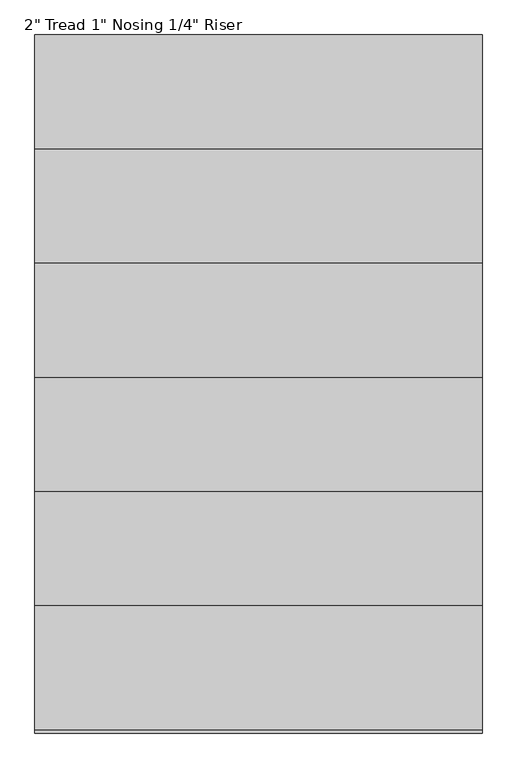
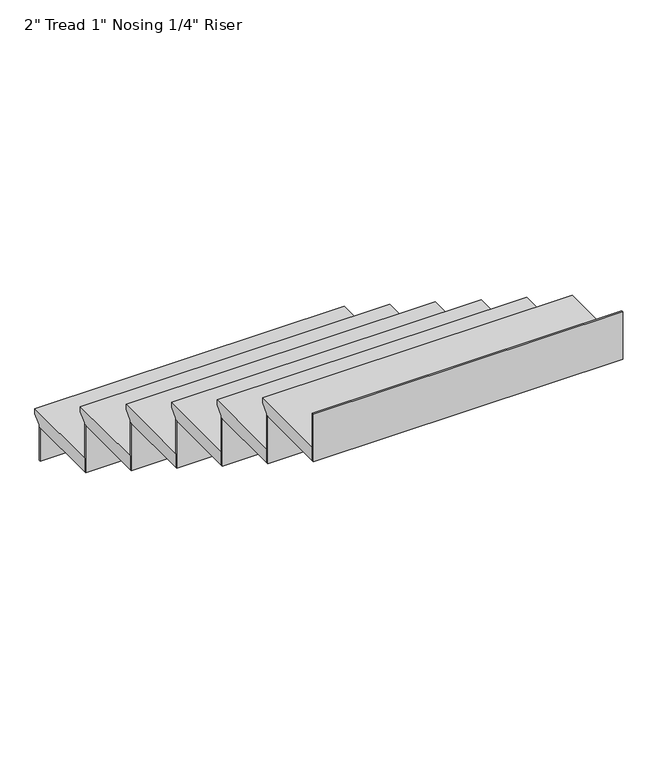
"""IFC4 building model written with IfcOpenShell, lengths in millimetres: stair flight geometry."""

from ifc_helpers import new_model, si_unit, frame, origin, place, context, project, spatial, polyline, outline, extrude, source, transform, mapped, element, save


def stair_flight_3c370561(model_context):
    return source(origin(), model_context, "Body", "SweptSolid", [
        extrude(outline(polyline([(16835.0111033, 2000.25), (17139.8111033, 2000.25), (17139.8111033, 1981.2), (17114.4111033, 1955.8), (17114.4111033, 1949.45), (16835.0111033, 1949.45), (16835.0111033, 2000.25)])), frame((-1579.5625, 0.0, 0.0), z_axis=(1.0, 0.0, 0.0), x_axis=(0.0, 1.0, 0.0)), (0.0, 0.0, 1.0), 1095.3438024),
        extrude(outline(polyline([(-1579.5625, 17108.0611033), (-1579.5625, 17114.4111033), (-484.2186975, 17114.4111033), (-484.2186975, 17108.0611033), (-1579.5625, 17108.0611033)])), frame((0.0, 0.0, 1822.45), z_axis=(0.0, 0.0, 1.0), x_axis=(1.0, 0.0, 0.0)), (0.0, 0.0, 1.0), 127.0),
        extrude(outline(polyline([(-1579.5625, 16828.6611033), (-1579.5625, 16835.0111033), (-484.2186975, 16835.0111033), (-484.2186975, 16828.6611033), (-1579.5625, 16828.6611033)])), frame((0.0, 0.0, 1949.45), z_axis=(0.0, 0.0, 1.0), x_axis=(1.0, 0.0, 0.0)), (0.0, 0.0, 1.0), 177.8),
        extrude(outline(polyline([(16555.6111033, 2178.05), (16860.4111033, 2178.05), (16860.4111033, 2159.0), (16835.0111033, 2133.6), (16835.0111033, 2127.25), (16555.6111033, 2127.25), (16555.6111033, 2178.05)])), frame((-1579.5625, 0.0, 0.0), z_axis=(1.0, 0.0, 0.0), x_axis=(0.0, 1.0, 0.0)), (0.0, 0.0, 1.0), 1095.3438024),
        extrude(outline(polyline([(-1579.5625, 16549.2611033), (-1579.5625, 16555.6111033), (-484.2186975, 16555.6111033), (-484.2186975, 16549.2611033), (-1579.5625, 16549.2611033)])), frame((0.0, 0.0, 2127.25), z_axis=(0.0, 0.0, 1.0), x_axis=(1.0, 0.0, 0.0)), (0.0, 0.0, 1.0), 177.8),
        extrude(outline(polyline([(16276.2111033, 2355.85), (16581.0111033, 2355.85), (16581.0111033, 2336.8), (16555.6111033, 2311.4), (16555.6111033, 2305.05), (16276.2111033, 2305.05), (16276.2111033, 2355.85)])), frame((-1579.5625, 0.0, 0.0), z_axis=(1.0, 0.0, 0.0), x_axis=(0.0, 1.0, 0.0)), (0.0, 0.0, 1.0), 1095.3438024),
        extrude(outline(polyline([(-1579.5625, 16269.8611033), (-1579.5625, 16276.2111033), (-484.2186975, 16276.2111033), (-484.2186975, 16269.8611033), (-1579.5625, 16269.8611033)])), frame((0.0, 0.0, 2305.05), z_axis=(0.0, 0.0, 1.0), x_axis=(1.0, 0.0, 0.0)), (0.0, 0.0, 1.0), 177.8),
        extrude(outline(polyline([(15996.8111033, 2533.65), (16301.6111033, 2533.65), (16301.6111033, 2514.6), (16276.2111033, 2489.2), (16276.2111033, 2482.85), (15996.8111033, 2482.85), (15996.8111033, 2533.65)])), frame((-1579.5625, 0.0, 0.0), z_axis=(1.0, 0.0, 0.0), x_axis=(0.0, 1.0, 0.0)), (0.0, 0.0, 1.0), 1095.3438024),
        extrude(outline(polyline([(-1579.5625, 15990.4611033), (-1579.5625, 15996.8111033), (-484.2186975, 15996.8111033), (-484.2186975, 15990.4611033), (-1579.5625, 15990.4611033)])), frame((0.0, 0.0, 2482.85), z_axis=(0.0, 0.0, 1.0), x_axis=(1.0, 0.0, 0.0)), (0.0, 0.0, 1.0), 177.8),
        extrude(outline(polyline([(15717.4111033, 2711.45), (16022.2111033, 2711.45), (16022.2111033, 2692.4), (15996.8111033, 2667.0), (15996.8111033, 2660.65), (15717.4111033, 2660.65), (15717.4111033, 2711.45)])), frame((-1579.5625, 0.0, 0.0), z_axis=(1.0, 0.0, 0.0), x_axis=(0.0, 1.0, 0.0)), (0.0, 0.0, 1.0), 1095.3438024),
        extrude(outline(polyline([(-1579.5625, 15711.0611033), (-1579.5625, 15717.4111033), (-484.2186975, 15717.4111033), (-484.2186975, 15711.0611033), (-1579.5625, 15711.0611033)])), frame((0.0, 0.0, 2660.65), z_axis=(0.0, 0.0, 1.0), x_axis=(1.0, 0.0, 0.0)), (0.0, 0.0, 1.0), 177.8),
        extrude(outline(polyline([(-1579.5625, 15431.6611033), (-1579.5625, 15438.0111033), (-484.2186975, 15438.0111033), (-484.2186975, 15431.6611033), (-1579.5625, 15431.6611033)])), frame((0.0, 0.0, 2838.45), z_axis=(0.0, 0.0, 1.0), x_axis=(1.0, 0.0, 0.0)), (0.0, 0.0, 1.0), 177.8),
        extrude(outline(polyline([(15438.0111033, 2889.25), (15742.8111033, 2889.25), (15742.8111033, 2870.2), (15717.4111033, 2844.8), (15717.4111033, 2838.45), (15438.0111033, 2838.45), (15438.0111033, 2889.25)])), frame((-1579.5625, 0.0, 0.0), z_axis=(1.0, 0.0, 0.0), x_axis=(0.0, 1.0, 0.0)), (0.0, 0.0, 1.0), 1095.3438024),
    ])


if __name__ == "__main__":
    model = new_model("IFC4")
    model_context = context("Model", 3, world=origin())
    ifc_project = project(units=[si_unit("LENGTHUNIT", "METRE", prefix="MILLI")], contexts=[model_context])
    site = spatial("IfcSite", under=ifc_project)
    building = spatial("IfcBuilding", under=site)
    placement = place(None, origin())
    stair_flight_shape = stair_flight_3c370561(model_context)
    element("IfcStairFlight", 1, ObjectType="2\" Tread 1\" Nosing 1/4\" Riser", at=placement, inside=building, context=model_context, shape_type="MappedRepresentation", body=[
        mapped(stair_flight_shape, transform((0.0, 0.0, 0.0), x_axis=(1.0, 0.0, 0.0), y_axis=(0.0, 1.0, 0.0), z_axis=(0.0, 0.0, 1.0))),
    ])
    save(model, "model.ifc")
